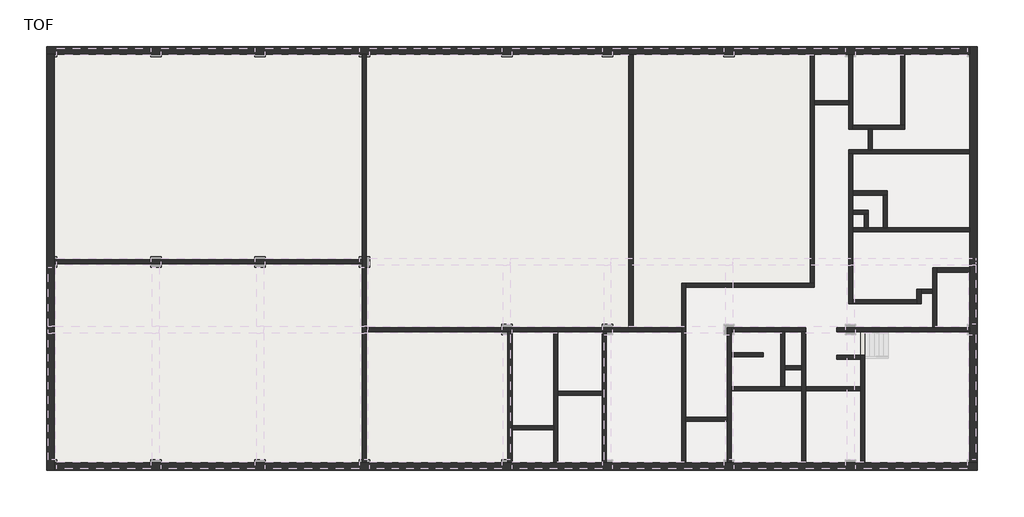
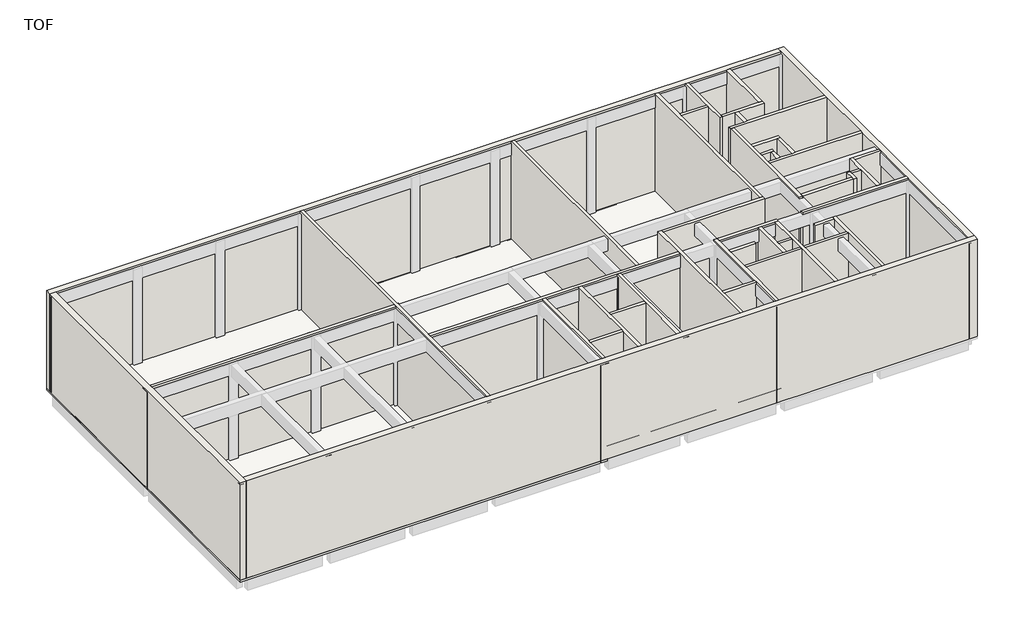
# One storey, part 1 of 3: 45 walls, 2 slabs.
"""IFC4 building model written with IfcOpenShell, lengths in millimetres."""

import ifcopenshell
import ifcopenshell.guid

model = None  # the IFC model being written
_history = None  # IfcOwnerHistory: only IFC2X3 demands one
_inside = {}  # id of a spatial element -> (the spatial element, [elements in it])
_under = {}  # id of a project, library or spatial element -> (it, [spatial elements below it])
_declared = {}  # id of a project -> (the project, [libraries it declares])
_typed = {}  # id of a type object -> (the type object, [elements of that type])
_made_of = {}  # id of a material, layer set ... -> (it, [elements and type objects made of it])


def new_model(schema):
    """Start an empty IFC model of exactly this schema.

    Asked for "IFC4X3", IfcOpenShell would pick the latest addendum, in which some entities
    have other attributes; the version numbers below select the first issue.
    IFC2X3 requires an IfcOwnerHistory on every rooted entity: one is made here for all.
    """
    global model, _history
    if schema == "IFC4X3":
        model = ifcopenshell.file(schema_version=(4, 3, 0, 0))
    else:
        model = ifcopenshell.file(schema=schema)
    _inside.clear()
    _under.clear()
    _declared.clear()
    _typed.clear()
    _made_of.clear()
    _history = None
    if model.schema == "IFC2X3":
        org = make("IfcOrganization", Name="unknown")
        user = make(
            "IfcPersonAndOrganization",
            ThePerson=make("IfcPerson", FamilyName="unknown"),
            TheOrganization=org,
        )
        app = make(
            "IfcApplication",
            ApplicationDeveloper=org,
            Version="unknown",
            ApplicationFullName="unknown",
            ApplicationIdentifier="unknown",
        )
        _history = make(
            "IfcOwnerHistory",
            OwningUser=user,
            OwningApplication=app,
            ChangeAction="ADDED",
            CreationDate=0,
        )
    return model


def make(cls, **values):
    """One entity of the class cls with the attributes given. An attribute that is None is left unset."""
    return model.create_entity(
        cls, **{name: value for name, value in values.items() if value is not None}
    )


def rooted(cls, **values):
    """An entity with a GlobalId (a new one), such as an element, a storey or a relation."""
    return make(cls, GlobalId=ifcopenshell.guid.new(), OwnerHistory=_history, **values)


def si_unit(unit_type, name, prefix=None):
    """IfcSIUnit, for example si_unit("LENGTHUNIT", "METRE", prefix="MILLI")."""
    return make("IfcSIUnit", UnitType=unit_type, Prefix=prefix, Name=name)


def assignment(units):
    """IfcUnitAssignment: the units of a project."""
    return None if units is None else make("IfcUnitAssignment", Units=units)


def point(xyz):
    """IfcCartesianPoint."""
    return None if xyz is None else make("IfcCartesianPoint", Coordinates=xyz)


def direction(xyz):
    """IfcDirection."""
    return None if xyz is None else make("IfcDirection", DirectionRatios=xyz)


def frame(location, z_axis=None, x_axis=None):
    """IfcAxis2Placement3D, a coordinate frame: its origin and axes. An axis left out is left unset."""
    return make(
        "IfcAxis2Placement3D",
        Location=point(location),
        Axis=direction(z_axis),
        RefDirection=direction(x_axis),
    )


def origin():
    """The frame at (0, 0, 0) with its axes left unset."""
    return frame((0.0, 0.0, 0.0))


def origin_with_axes():
    """The frame at (0, 0, 0) with the z axis (0, 0, 1) and the x axis (1, 0, 0) written out."""
    return frame((0.0, 0.0, 0.0), z_axis=(0.0, 0.0, 1.0), x_axis=(1.0, 0.0, 0.0))


def place(relative_to, where):
    """IfcLocalPlacement: puts the frame where relative to a parent placement (None: the world)."""
    return make(
        "IfcLocalPlacement", PlacementRelTo=relative_to, RelativePlacement=where
    )


def context(
    kind, dimensions, precision=None, world=None, true_north=None, identifier=None
):
    """IfcGeometricRepresentationContext, for example the 3D "Model" context."""
    return make(
        "IfcGeometricRepresentationContext",
        ContextIdentifier=identifier,
        ContextType=kind,
        CoordinateSpaceDimension=dimensions,
        Precision=precision,
        WorldCoordinateSystem=world,
        TrueNorth=true_north,
    )


def project(units=None, contexts=None):
    """IfcProject with its units and contexts."""
    return rooted(
        "IfcProject",
        Name="project",
        RepresentationContexts=contexts,
        UnitsInContext=assignment(units),
    )


def spatial(cls, under=None, at=None, **own):
    """A site, building, storey or space (cls), placed at a placement, below another one or the project."""
    s = rooted(cls, ObjectPlacement=at, **own)
    if under is not None:
        _under.setdefault(under.id(), (under, []))[1].append(s)
    return s


def polyline(points):
    """IfcPolyline through the points."""
    return make("IfcPolyline", Points=[point(p) for p in points])


def outline(outer, holes=None, kind="AREA"):
    """IfcArbitraryClosedProfileDef: a profile drawn as a closed curve; with holes, ...WithVoids."""
    if holes is None:
        return make("IfcArbitraryClosedProfileDef", ProfileType=kind, OuterCurve=outer)
    return make(
        "IfcArbitraryProfileDefWithVoids",
        ProfileType=kind,
        OuterCurve=outer,
        InnerCurves=holes,
    )


def extrude(swept, where, along, depth):
    """IfcExtrudedAreaSolid: the profile swept, set in the frame where, extruded along a direction by depth."""
    return make(
        "IfcExtrudedAreaSolid",
        SweptArea=swept,
        Position=where,
        ExtrudedDirection=direction(along),
        Depth=depth,
    )


def faces_of(points, faces, orient=None, outer=None):
    """IfcFace entities. A face is a list of loops; a loop is a list of indices into points, from 0.

    orient and outer hold one flag for each loop. By default every Orientation is true, the
    first loop of a face is its IfcFaceOuterBound and the others are IfcFaceBound.
    """
    made = []
    for i, loops in enumerate(faces):
        bounds = []
        for j, loop in enumerate(loops):
            is_outer = j == 0 if outer is None else outer[i][j]
            bounds.append(
                make(
                    "IfcFaceOuterBound" if is_outer else "IfcFaceBound",
                    Bound=make("IfcPolyLoop", Polygon=[points[k] for k in loop]),
                    Orientation=True if orient is None else orient[i][j],
                )
            )
        made.append(make("IfcFace", Bounds=bounds))
    return made


def faceted_brep(points, faces, orient=None, outer=None, voids=None):
    """IfcFacetedBrep: a solid bounded by flat faces; with voids (closed shells), ...WithVoids."""
    shared = [point(p) for p in points]
    hull = make("IfcClosedShell", CfsFaces=faces_of(shared, faces, orient, outer))
    if voids is None:
        return make("IfcFacetedBrep", Outer=hull)
    return make(
        "IfcFacetedBrepWithVoids",
        Outer=hull,
        Voids=[
            make(cls, CfsFaces=faces_of(shared, fs, o, b)) for cls, fs, o, b in voids
        ],
    )


def shape(context_of_items, identifier, shape_type, items):
    """IfcShapeRepresentation: the items that make up one representation, for example the "Body"."""
    return make(
        "IfcShapeRepresentation",
        ContextOfItems=context_of_items,
        RepresentationIdentifier=identifier,
        RepresentationType=shape_type,
        Items=items,
    )


def made_of(thing, what):
    """Note that an element or type object is made of a material, layer set ...; save() writes the relation."""
    if what is not None:
        _made_of.setdefault(what.id(), (what, []))[1].append(thing)
    return thing


def element(
    cls,
    number,
    at=None,
    inside=None,
    cuts=None,
    type_object=None,
    material=None,
    context=None,
    identifier="Body",
    shape_type=None,
    held_by="IfcProductDefinitionShape",
    body=None,
    shapes=None,
    **own,
):
    """One element of the class cls, such as IfcWall. Its Tag is "e" and its number.

    at: its placement. inside: the storey or other place that contains it. cuts: it is an
    opening in that element (IfcRelVoidsElement). A single representation is given by context,
    identifier, shape_type and body (its items); several are given by shapes. held_by: the class
    of the entity that holds the representations. save() writes the other relations.
    """
    e = rooted(cls, Tag="e%d" % number, ObjectPlacement=at, **own)
    if body is not None:
        shapes = [shape(context, identifier, shape_type, body)]
    if shapes is not None:
        e.Representation = make(held_by, Representations=shapes)
    if inside is not None:
        _inside.setdefault(inside.id(), (inside, []))[1].append(e)
    if cuts is not None:
        rooted(
            "IfcRelVoidsElement", RelatingBuildingElement=cuts, RelatedOpeningElement=e
        )
    if type_object is not None:
        _typed.setdefault(type_object.id(), (type_object, []))[1].append(e)
    return made_of(e, material)


def aggregate(whole, parts):
    """IfcRelAggregates: a whole, such as a stair, and the parts it consists of."""
    return rooted("IfcRelAggregates", RelatingObject=whole, RelatedObjects=parts)


def save(model, path):
    """Write the relations noted so far, then the file.

    IfcRelAggregates (storeys below a building ...), IfcRelContainedInSpatialStructure (elements
    in a storey), IfcRelDefinesByType, IfcRelAssociatesMaterial and IfcRelDeclares: one each for
    every whole, place, type object, material and project.
    """
    for whole, parts in _under.values():
        aggregate(whole, parts)
    for where, things in _inside.values():
        rooted(
            "IfcRelContainedInSpatialStructure",
            RelatedElements=things,
            RelatingStructure=where,
        )
    for kind, things in _typed.values():
        rooted("IfcRelDefinesByType", RelatedObjects=things, RelatingType=kind)
    for what, things in _made_of.values():
        rooted("IfcRelAssociatesMaterial", RelatedObjects=things, RelatingMaterial=what)
    for by, libraries in _declared.values():
        rooted("IfcRelDeclares", RelatingContext=by, RelatedDefinitions=libraries)
    model.write(path)


model = new_model("IFC4")

# Units and contexts
model_context = context("Model", 3, world=origin())
ifc_project = project(units=[si_unit("LENGTHUNIT", "METRE", prefix="MILLI")], contexts=[model_context])

# Site, building, storey
site = spatial("IfcSite", under=ifc_project)
building = spatial("IfcBuilding", under=site)
storey = spatial("IfcBuildingStorey", under=building, Name="TOF", Elevation=150.0)

# Slabs
placement = place(None, origin())
element("IfcSlab", 1, ObjectType="H_FL_AMF_RC Slab_T150", at=placement, inside=storey, context=model_context, shape_type="Brep", body=[
    faceted_brep([(-375.3, 24716.5208589, 0.0), (43724.7, 24716.5208589, 0.0), (43724.7, 10966.5208589, 0.0), (36324.7, 10966.5208589, 0.0), (36324.7, 8416.5208589, 0.0), (32224.7, 8416.5208589, 0.0), (31624.7, 8416.5208589, 0.0), (26424.7, 8416.5208589, 0.0), (25824.7, 8416.5208589, 0.0), (17924.7, 8416.5208589, 0.0), (17924.7, 12016.5208589, 0.0), (17924.7, 12316.5208589, 0.0), (17624.7, 12316.5208589, 0.0), (12224.7, 12316.5208589, 0.0), (11624.7, 12316.5208589, 0.0), (6224.7, 12316.5208589, 0.0), (5624.7, 12316.5208589, 0.0), (224.7, 12316.5208589, 0.0), (-375.3, 12316.5208589, 0.0), (-375.3, 24716.5208589, 150.0), (-375.3, 24116.5208589, 150.0), (-375.3, 12616.5208589, 150.0), (-375.3, 12316.5208589, 150.0), (224.7, 12316.5208589, 150.0), (5624.7, 12316.5208589, 150.0), (6224.7, 12316.5208589, 150.0), (11624.7, 12316.5208589, 150.0), (12224.7, 12316.5208589, 150.0), (17624.7, 12316.5208589, 150.0), (17924.7, 12316.5208589, 150.0), (17924.7, 12016.5208589, 150.0), (17924.7, 8416.5208589, 150.0), (25824.7, 8416.5208589, 150.0), (26424.7, 8416.5208589, 150.0), (31624.7, 8416.5208589, 150.0), (32224.7, 8416.5208589, 150.0), (36324.7, 8416.5208589, 150.0), (36324.7, 10966.5208589, 150.0), (43724.7, 10966.5208589, 150.0), (43724.7, 24716.5208589, 150.0), (39224.7, 24716.5208589, 150.0), (38624.7, 24716.5208589, 150.0), (32224.7, 24716.5208589, 150.0), (31624.7, 24716.5208589, 150.0), (26424.7, 24716.5208589, 150.0), (25824.7, 24716.5208589, 150.0), (18224.7, 24716.5208589, 150.0), (17624.7, 24716.5208589, 150.0), (12224.7, 24716.5208589, 150.0), (11624.7, 24716.5208589, 150.0), (6224.7, 24716.5208589, 150.0), (5624.7, 24716.5208589, 150.0), (224.7, 24716.5208589, 150.0)], [[[0, 1, 2, 3, 4, 5, 6, 7, 8, 9, 10, 11, 12, 13, 14, 15, 16, 17, 18]], [[19, 20, 21, 22, 23, 24, 25, 26, 27, 28, 29, 30, 31, 32, 33, 34, 35, 36, 37, 38, 39, 40, 41, 42, 43, 44, 45, 46, 47, 48, 49, 50, 51, 52]], [[0, 18, 22, 21, 20, 19]], [[1, 0, 19, 52, 51, 50, 49, 48, 47, 46, 45, 44, 43, 42, 41, 40, 39]], [[2, 1, 39, 38]], [[3, 2, 38, 37]], [[4, 3, 37, 36]], [[9, 8, 7, 6, 5, 4, 36, 35, 34, 33, 32, 31]], [[11, 10, 9, 31, 30, 29]], [[18, 17, 16, 15, 14, 13, 12, 11, 29, 28, 27, 26, 25, 24, 23, 22]]]),
])
element("IfcSlab", 2, ObjectType="H_FL_AMF_RC Slab_T150", at=placement, inside=storey, context=model_context, shape_type="SweptSolid", body=[
    extrude(outline(polyline([(17924.7, 12316.5208589), (17924.7, 8416.5208589), (26307.7, 8416.5208589), (26307.7, 316.5208589), (-375.3, 316.5208589), (-375.3, 12316.5208589), (17924.7, 12316.5208589)])), origin_with_axes(), (0.0, 0.0, 1.0), 150.0),
])

# Walls
element("IfcWall", 3, ObjectType="H_WA_AMW_Brick Wall_Ext (0.5B_50_1.0B / Emulsion)", at=placement, inside=storey, context=model_context, shape_type="Brep", body=[
    faceted_brep([(-375.3, 24286.5208589, 150.0), (54.7, 24286.5208589, 150.0), (17807.7, 24286.5208589, 150.0), (18041.7, 24286.5208589, 150.0), (33157.7, 24286.5208589, 150.0), (33391.7, 24286.5208589, 150.0), (43607.7, 24286.5208589, 150.0), (43841.7, 24286.5208589, 150.0), (52794.7, 24286.5208589, 150.0), (52794.7, 24286.5208589, 7650.0), (49041.7, 24286.5208589, 7650.0), (48807.7, 24286.5208589, 7650.0), (46041.7, 24286.5208589, 7650.0), (45807.7, 24286.5208589, 7650.0), (43841.7, 24286.5208589, 7650.0), (43607.7, 24286.5208589, 7650.0), (33391.7, 24286.5208589, 7650.0), (33157.7, 24286.5208589, 7650.0), (18041.7, 24286.5208589, 7650.0), (17807.7, 24286.5208589, 7650.0), (54.7, 24286.5208589, 7650.0), (-375.3, 24286.5208589, 7650.0), (-375.3, 24716.5208589, 150.0), (-375.3, 24716.5208589, 7650.0), (52794.7, 24716.5208589, 7650.0), (52794.7, 24716.5208589, 150.0)], [[[0, 1, 2, 3, 4, 5, 6, 7, 8, 9, 10, 11, 12, 13, 14, 15, 16, 17, 18, 19, 20, 21]], [[22, 23, 24, 25]], [[8, 7, 6, 5, 4, 3, 2, 1, 0, 22, 25]], [[21, 20, 19, 18, 17, 16, 15, 14, 13, 12, 11, 10, 9, 24, 23]], [[0, 21, 23, 22]], [[9, 8, 25, 24]]]),
])
element("IfcWall", 4, ObjectType="H_WA_AMW_Brick Wall_Ext (0.5B_50_1.0B / Emulsion)", at=placement, inside=storey, context=model_context, shape_type="Brep", body=[
    faceted_brep([(54.7, 316.5208589, 150.0), (54.7, 746.5208589, 150.0), (54.7, 12199.5208589, 150.0), (54.7, 12433.5208589, 150.0), (54.7, 24286.5208589, 150.0), (54.7, 24286.5208589, 7650.0), (54.7, 12433.5208589, 7650.0), (54.7, 12199.5208589, 7650.0), (54.7, 746.5208589, 7650.0), (54.7, 316.5208589, 7650.0), (-375.3, 316.5208589, 150.0), (-375.3, 316.5208589, 7650.0), (-375.3, 24286.5208589, 7650.0), (-375.3, 24286.5208589, 150.0)], [[[0, 1, 2, 3, 4, 5, 6, 7, 8, 9]], [[10, 11, 12, 13]], [[4, 3, 2, 1, 0, 10, 13]], [[9, 8, 7, 6, 5, 12, 11]], [[0, 9, 11, 10]], [[5, 4, 13, 12]]]),
])
element("IfcWall", 5, ObjectType="H_WA_AMW_Brick Wall_Ext (0.5B_50_1.0B / Emulsion)", at=placement, inside=storey, context=model_context, shape_type="Brep", body=[
    faceted_brep([(53224.7, 746.5208589, 150.0), (52794.7, 746.5208589, 150.0), (46741.7, 746.5208589, 150.0), (46507.7, 746.5208589, 150.0), (43341.7, 746.5208589, 150.0), (43107.7, 746.5208589, 150.0), (39041.7, 746.5208589, 150.0), (38807.7, 746.5208589, 150.0), (26424.7, 746.5208589, 150.0), (26190.7, 746.5208589, 150.0), (18041.7, 746.5208589, 150.0), (17807.7, 746.5208589, 150.0), (54.7, 746.5208589, 150.0), (54.7, 746.5208589, 7650.0), (17807.7, 746.5208589, 7650.0), (18041.7, 746.5208589, 7650.0), (26190.7, 746.5208589, 7650.0), (26424.7, 746.5208589, 7650.0), (28824.7, 746.5208589, 7650.0), (29058.7, 746.5208589, 7650.0), (31624.7, 746.5208589, 7650.0), (31858.7, 746.5208589, 7650.0), (36207.7, 746.5208589, 7650.0), (36441.7, 746.5208589, 7650.0), (38807.7, 746.5208589, 7650.0), (39041.7, 746.5208589, 7650.0), (43107.7, 746.5208589, 7650.0), (43341.7, 746.5208589, 7650.0), (46507.7, 746.5208589, 7650.0), (46741.7, 746.5208589, 7650.0), (52794.7, 746.5208589, 7650.0), (53224.7, 746.5208589, 7650.0), (53224.7, 316.5208589, 150.0), (53224.7, 316.5208589, 7650.0), (54.7, 316.5208589, 7650.0), (54.7, 316.5208589, 150.0)], [[[0, 1, 2, 3, 4, 5, 6, 7, 8, 9, 10, 11, 12, 13, 14, 15, 16, 17, 18, 19, 20, 21, 22, 23, 24, 25, 26, 27, 28, 29, 30, 31]], [[32, 33, 34, 35]], [[12, 11, 10, 9, 8, 7, 6, 5, 4, 3, 2, 1, 0, 32, 35]], [[31, 30, 29, 28, 27, 26, 25, 24, 23, 22, 21, 20, 19, 18, 17, 16, 15, 14, 13, 34, 33]], [[0, 31, 33, 32]], [[13, 12, 35, 34]]]),
])
element("IfcWall", 6, ObjectType="H_WA_AMW_Brick Wall_Ext (0.5B_50_1.0B / Emulsion)", at=placement, inside=storey, context=model_context, shape_type="Brep", body=[
    faceted_brep([(52794.7, 24716.5208589, 150.0), (52794.7, 24286.5208589, 150.0), (52794.7, 8533.5208589, 150.0), (52794.7, 8299.5208589, 150.0), (52794.7, 746.5208589, 150.0), (52794.7, 746.5208589, 7650.0), (52794.7, 8299.5208589, 7650.0), (52794.7, 8533.5208589, 7650.0), (52794.7, 11733.5208589, 7650.0), (52794.7, 11967.5208589, 7650.0), (52794.7, 14049.5208589, 7650.0), (52794.7, 14283.5208589, 7650.0), (52794.7, 18549.5208589, 7650.0), (52794.7, 18783.5208589, 7650.0), (52794.7, 24286.5208589, 7650.0), (52794.7, 24716.5208589, 7650.0), (53224.7, 24716.5208589, 150.0), (53224.7, 24716.5208589, 7650.0), (53224.7, 746.5208589, 7650.0), (53224.7, 746.5208589, 150.0)], [[[0, 1, 2, 3, 4, 5, 6, 7, 8, 9, 10, 11, 12, 13, 14, 15]], [[16, 17, 18, 19]], [[4, 3, 2, 1, 0, 16, 19]], [[15, 14, 13, 12, 11, 10, 9, 8, 7, 6, 5, 18, 17]], [[0, 15, 17, 16]], [[5, 4, 19, 18]]]),
])
element("IfcWall", 7, ObjectType="H_WA_AMW_Block Wall_Int_T200 (Both Plaster_Emulsion)", at=placement, inside=storey, context=model_context, shape_type="SweptSolid", body=[
    extrude(outline(polyline([(17807.7, 12199.5208589), (54.7, 12199.5208589), (54.7, 12433.5208589), (17807.7, 12433.5208589), (17807.7, 12199.5208589)])), frame((0.0, 0.0, 150.0), z_axis=(0.0, 0.0, 1.0), x_axis=(1.0, 0.0, 0.0)), (0.0, 0.0, 1.0), 7500.0),
])
element("IfcWall", 8, ObjectType="H_WA_AMW_Block Wall_Int_T200 (Both Plaster_Emulsion)", at=placement, inside=storey, context=model_context, shape_type="Brep", body=[
    faceted_brep([(17807.7, 24286.5208589, 150.0), (17807.7, 12433.5208589, 150.0), (17807.7, 12199.5208589, 150.0), (17807.7, 746.5208589, 150.0), (17807.7, 746.5208589, 7650.0), (17807.7, 12199.5208589, 7650.0), (17807.7, 12433.5208589, 7650.0), (17807.7, 24286.5208589, 7650.0), (18041.7, 24286.5208589, 150.0), (18041.7, 24286.5208589, 7650.0), (18041.7, 8533.5208589, 7650.0), (18041.7, 8299.5208589, 7650.0), (18041.7, 746.5208589, 7650.0), (18041.7, 746.5208589, 150.0), (18041.7, 8299.5208589, 150.0), (18041.7, 8533.5208589, 150.0)], [[[0, 1, 2, 3, 4, 5, 6, 7]], [[8, 9, 10, 11, 12, 13, 14, 15]], [[3, 2, 1, 0, 8, 15, 14, 13]], [[7, 6, 5, 4, 12, 11, 10, 9]], [[0, 7, 9, 8]], [[4, 3, 13, 12]]]),
])
element("IfcWall", 9, ObjectType="H_WA_AMW_Block Wall_Int_T200 (Both Plaster_Emulsion)", at=placement, inside=storey, context=model_context, shape_type="SweptSolid", body=[
    extrude(outline(polyline([(33157.7, 8533.5208589), (33157.7, 24286.5208589), (33391.7, 24286.5208589), (33391.7, 8533.5208589), (33157.7, 8533.5208589)])), frame((0.0, 0.0, 150.0), z_axis=(0.0, 0.0, 1.0), x_axis=(1.0, 0.0, 0.0)), (0.0, 0.0, 1.0), 7500.0),
])
element("IfcWall", 10, ObjectType="H_WA_AMW_Block Wall_Int_T200 (Both Plaster_Emulsion)", at=placement, inside=storey, context=model_context, shape_type="Brep", body=[
    faceted_brep([(18041.7, 8299.5208589, 150.0), (26190.7, 8299.5208589, 150.0), (26424.7, 8299.5208589, 150.0), (36207.7, 8299.5208589, 150.0), (36207.7, 8299.5208589, 7650.0), (31858.7, 8299.5208589, 7650.0), (31624.7, 8299.5208589, 7650.0), (29058.7, 8299.5208589, 7650.0), (28824.7, 8299.5208589, 7650.0), (26424.7, 8299.5208589, 7650.0), (26190.7, 8299.5208589, 7650.0), (18041.7, 8299.5208589, 7650.0), (18041.7, 8533.5208589, 150.0), (18041.7, 8533.5208589, 7650.0), (33157.7, 8533.5208589, 7650.0), (33391.7, 8533.5208589, 7650.0), (36207.7, 8533.5208589, 7650.0), (36207.7, 8533.5208589, 150.0), (33391.7, 8533.5208589, 150.0), (33157.7, 8533.5208589, 150.0)], [[[0, 1, 2, 3, 4, 5, 6, 7, 8, 9, 10, 11]], [[12, 13, 14, 15, 16, 17, 18, 19]], [[3, 2, 1, 0, 12, 19, 18, 17]], [[11, 10, 9, 8, 7, 6, 5, 4, 16, 15, 14, 13]], [[0, 11, 13, 12]], [[4, 3, 17, 16]]]),
])
element("IfcWall", 11, ObjectType="H_WA_AMW_Block Wall_Int_T200 (Both Plaster_Emulsion)", at=placement, inside=storey, context=model_context, shape_type="Brep", body=[
    faceted_brep([(36207.7, 11083.5208589, 1150.0), (36207.7, 746.5208589, 1150.0), (36207.7, 746.5208589, 7650.0), (36207.7, 8299.5208589, 7650.0), (36207.7, 8533.5208589, 7650.0), (36207.7, 11083.5208589, 7650.0), (36441.7, 11083.5208589, 1150.0), (36441.7, 11083.5208589, 7650.0), (36441.7, 10849.5208589, 7650.0), (36441.7, 3380.5208589, 7650.0), (36441.7, 3146.5208589, 7650.0), (36441.7, 746.5208589, 7650.0), (36441.7, 746.5208589, 1150.0), (36441.7, 3146.5208589, 1150.0), (36441.7, 3380.5208589, 1150.0)], [[[0, 1, 2, 3, 4, 5]], [[6, 7, 8, 9, 10, 11, 12, 13, 14]], [[1, 0, 6, 14, 13, 12]], [[5, 4, 3, 2, 11, 10, 9, 8, 7]], [[2, 1, 12, 11]], [[0, 5, 7, 6]]]),
])
element("IfcWall", 12, ObjectType="H_WA_AMW_Block Wall_Int_T200 (Both Plaster_Emulsion)", at=placement, inside=storey, context=model_context, shape_type="Brep", body=[
    faceted_brep([(36441.7, 10849.5208589, 150.0), (43841.7, 10849.5208589, 150.0), (43841.7, 10849.5208589, 7650.0), (36441.7, 10849.5208589, 7650.0), (36441.7, 11083.5208589, 150.0), (36441.7, 11083.5208589, 1150.0), (36441.7, 11083.5208589, 7650.0), (43607.7, 11083.5208589, 7650.0), (43841.7, 11083.5208589, 7650.0), (43841.7, 11083.5208589, 150.0), (43607.7, 11083.5208589, 150.0)], [[[0, 1, 2, 3]], [[4, 5, 6, 7, 8, 9, 10]], [[1, 0, 4, 10, 9]], [[3, 2, 8, 7, 6]], [[0, 3, 6, 5, 4]], [[2, 1, 9, 8]]]),
])
element("IfcWall", 13, ObjectType="H_WA_AMW_Block Wall_Int_T200 (Both Plaster_Emulsion)", at=placement, inside=storey, context=model_context, shape_type="Brep", body=[
    faceted_brep([(43841.7, 11083.5208589, 150.0), (43841.7, 24286.5208589, 150.0), (43841.7, 24286.5208589, 7650.0), (43841.7, 21586.5208589, 7650.0), (43841.7, 21352.5208589, 7650.0), (43841.7, 11083.5208589, 7650.0), (43607.7, 11083.5208589, 150.0), (43607.7, 11083.5208589, 7650.0), (43607.7, 24286.5208589, 7650.0), (43607.7, 24286.5208589, 150.0)], [[[0, 1, 2, 3, 4, 5]], [[6, 7, 8, 9]], [[1, 0, 6, 9]], [[5, 4, 3, 2, 8, 7]], [[0, 5, 7, 6]], [[2, 1, 9, 8]]]),
])
element("IfcWall", 14, ObjectType="H_WA_AMW_Block Wall_Int_T200 (Both Plaster_Emulsion)", at=placement, inside=storey, context=model_context, shape_type="SweptSolid", body=[
    extrude(outline(polyline([(45807.7, 21352.5208589), (43841.7, 21352.5208589), (43841.7, 21586.5208589), (45807.7, 21586.5208589), (45807.7, 21352.5208589)])), frame((0.0, 0.0, 1150.0), z_axis=(0.0, 0.0, 1.0), x_axis=(1.0, 0.0, 0.0)), (0.0, 0.0, 1.0), 6500.0),
])
element("IfcWall", 15, ObjectType="H_WA_AMW_Block Wall_Int_T200 (Both Plaster_Emulsion)", at=placement, inside=storey, context=model_context, shape_type="Brep", body=[
    faceted_brep([(45807.7, 24286.5208589, 1150.0), (45807.7, 21586.5208589, 1150.0), (45807.7, 21352.5208589, 1150.0), (45807.7, 19949.5208589, 1150.0), (45807.7, 19949.5208589, 7650.0), (45807.7, 21352.5208589, 7650.0), (45807.7, 21586.5208589, 7650.0), (45807.7, 24286.5208589, 7650.0), (46041.7, 24286.5208589, 1150.0), (46041.7, 24286.5208589, 7650.0), (46041.7, 20183.5208589, 7650.0), (46041.7, 19949.5208589, 7650.0), (46041.7, 19949.5208589, 1150.0), (46041.7, 20183.5208589, 1150.0)], [[[0, 1, 2, 3, 4, 5, 6, 7]], [[8, 9, 10, 11, 12, 13]], [[3, 2, 1, 0, 8, 13, 12]], [[7, 6, 5, 4, 11, 10, 9]], [[0, 7, 9, 8]], [[4, 3, 12, 11]]]),
])
element("IfcWall", 16, ObjectType="H_WA_AMW_Block Wall_Int_T200 (Both Plaster_Emulsion)", at=placement, inside=storey, context=model_context, shape_type="SweptSolid", body=[
    extrude(outline(polyline([(49743.7, 9899.5208589), (46041.7, 9899.5208589), (46041.7, 10133.5208589), (49743.7, 10133.5208589), (49743.7, 9899.5208589)])), frame((0.0, 0.0, 1150.0), z_axis=(0.0, 0.0, 1.0), x_axis=(1.0, 0.0, 0.0)), (0.0, 0.0, 1.0), 6500.0),
])
element("IfcWall", 17, ObjectType="H_WA_AMW_Block Wall_Int_T200 (Both Plaster_Emulsion)", at=placement, inside=storey, context=model_context, shape_type="Brep", body=[
    faceted_brep([(50660.7, 11967.5208589, 150.0), (50660.7, 8533.5208589, 150.0), (50660.7, 8533.5208589, 7650.0), (50660.7, 10499.5208589, 7650.0), (50660.7, 10733.5208589, 7650.0), (50660.7, 11967.5208589, 7650.0), (50894.7, 11967.5208589, 150.0), (50894.7, 11967.5208589, 1150.0), (50894.7, 11967.5208589, 7650.0), (50894.7, 11733.5208589, 7650.0), (50894.7, 8533.5208589, 7650.0), (50894.7, 8533.5208589, 150.0)], [[[0, 1, 2, 3, 4, 5]], [[6, 7, 8, 9, 10, 11]], [[1, 0, 6, 11]], [[5, 4, 3, 2, 10, 9, 8]], [[0, 5, 8, 7, 6]], [[2, 1, 11, 10]]]),
])
element("IfcWall", 18, ObjectType="H_WA_AMW_Block Wall_Int_T200 (Both Plaster_Emulsion)", at=placement, inside=storey, context=model_context, shape_type="SweptSolid", body=[
    extrude(outline(polyline([(52794.7, 11733.5208589), (50894.7, 11733.5208589), (50894.7, 11967.5208589), (52794.7, 11967.5208589), (52794.7, 11733.5208589)])), frame((0.0, 0.0, 1150.0), z_axis=(0.0, 0.0, 1.0), x_axis=(1.0, 0.0, 0.0)), (0.0, 0.0, 1.0), 6500.0),
])
element("IfcWall", 19, ObjectType="H_WA_AMW_Block Wall_Int_T200 (Both Plaster_Emulsion)", at=placement, inside=storey, context=model_context, shape_type="Brep", body=[
    faceted_brep([(49977.7, 9899.5208589, 1150.0), (49977.7, 10499.5208589, 1150.0), (49977.7, 10733.5208589, 1150.0), (49977.7, 10733.5208589, 7650.0), (49977.7, 10499.5208589, 7650.0), (49977.7, 9899.5208589, 7650.0), (49743.7, 9899.5208589, 1150.0), (49743.7, 9899.5208589, 7650.0), (49743.7, 10133.5208589, 7650.0), (49743.7, 10733.5208589, 7650.0), (49743.7, 10733.5208589, 1150.0), (49743.7, 10133.5208589, 1150.0)], [[[0, 1, 2, 3, 4, 5]], [[6, 7, 8, 9, 10, 11]], [[2, 1, 0, 6, 11, 10]], [[5, 4, 3, 9, 8, 7]], [[3, 2, 10, 9]], [[0, 5, 7, 6]]]),
])
element("IfcWall", 20, ObjectType="H_WA_AMW_Block Wall_Int_T200 (Both Plaster_Emulsion)", at=placement, inside=storey, context=model_context, shape_type="SweptSolid", body=[
    extrude(outline(polyline([(50660.7, 10499.5208589), (49977.7, 10499.5208589), (49977.7, 10733.5208589), (50660.7, 10733.5208589), (50660.7, 10499.5208589)])), frame((0.0, 0.0, 1150.0), z_axis=(0.0, 0.0, 1.0), x_axis=(1.0, 0.0, 0.0)), (0.0, 0.0, 1.0), 6500.0),
])
element("IfcWall", 21, ObjectType="H_WA_AMW_Block Wall_Int_T200 (Both Plaster_Emulsion)", at=placement, inside=storey, context=model_context, shape_type="Brep", body=[
    faceted_brep([(46507.7, 6933.5208589, 7650.0), (46507.7, 6933.5208589, 1250.0), (46507.7, 6933.5208589, 150.0), (46507.7, 6699.5208589, 150.0), (46507.7, 5130.5208589, 150.0), (46507.7, 4896.5208589, 150.0), (46507.7, 746.5208589, 150.0), (46507.7, 746.5208589, 7650.0), (46507.7, 4896.5208589, 7650.0), (46507.7, 5130.5208589, 7650.0), (46507.7, 6699.5208589, 7650.0), (46741.7, 6933.5208589, 150.0), (46741.7, 6933.5208589, 1250.0), (46741.7, 6933.5208589, 7650.0), (46741.7, 746.5208589, 7650.0), (46741.7, 746.5208589, 150.0)], [[[0, 1, 2, 3, 4, 5, 6, 7, 8, 9, 10]], [[11, 12, 13, 14, 15]], [[6, 5, 4, 3, 2, 11, 15]], [[0, 10, 9, 8, 7, 14, 13]], [[7, 6, 15, 14]], [[0, 13, 12, 11, 2, 1]]]),
])
element("IfcWall", 22, ObjectType="H_WA_AMW_Block Wall_Int_T200 (Both Plaster_Emulsion)", at=placement, inside=storey, context=model_context, shape_type="SweptSolid", body=[
    extrude(outline(polyline([(46507.7, 6699.5208589), (45124.7, 6699.5208589), (45124.7, 6933.5208589), (46507.7, 6933.5208589), (46507.7, 6699.5208589)])), frame((0.0, 0.0, 150.0), z_axis=(0.0, 0.0, 1.0), x_axis=(1.0, 0.0, 0.0)), (0.0, 0.0, 1.0), 7500.0),
])
element("IfcWall", 23, ObjectType="H_WA_AMW_Block Wall_Int_T200 (Both Plaster_Emulsion)", at=placement, inside=storey, context=model_context, shape_type="Brep", body=[
    faceted_brep([(52794.7, 8533.5208589, 150.0), (50894.7, 8533.5208589, 150.0), (50660.7, 8533.5208589, 150.0), (45124.7, 8533.5208589, 150.0), (45124.7, 8533.5208589, 7650.0), (50660.7, 8533.5208589, 7650.0), (50894.7, 8533.5208589, 7650.0), (52794.7, 8533.5208589, 7650.0), (52794.7, 8299.5208589, 150.0), (52794.7, 8299.5208589, 7650.0), (45124.7, 8299.5208589, 7650.0), (45124.7, 8299.5208589, 150.0), (46507.7, 8299.5208589, 150.0), (46741.7, 8299.5208589, 150.0)], [[[0, 1, 2, 3, 4, 5, 6, 7]], [[8, 9, 10, 11, 12, 13]], [[3, 2, 1, 0, 8, 13, 12, 11]], [[4, 3, 11, 10]], [[7, 6, 5, 4, 10, 9]], [[0, 7, 9, 8]]]),
])
element("IfcWall", 24, ObjectType="H_WA_AMW_Block Wall_Int_T200 (Both Plaster_Emulsion)", at=placement, inside=storey, context=model_context, shape_type="Brep", body=[
    faceted_brep([(38807.7, 8533.5208589, 150.0), (38807.7, 746.5208589, 150.0), (38807.7, 746.5208589, 1000.0), (38807.7, 8533.5208589, 1000.0), (38807.7, 746.5208589, 7650.0), (38807.7, 3146.5208589, 7650.0), (38807.7, 3380.5208589, 7650.0), (38807.7, 8533.5208589, 7650.0), (38807.7, 8533.5208589, 1150.0), (38807.7, 3380.5208589, 1150.0), (38807.7, 3146.5208589, 1150.0), (38807.7, 746.5208589, 1150.0), (39041.7, 746.5208589, 150.0), (39041.7, 4896.5208589, 150.0), (39041.7, 5130.5208589, 150.0), (39041.7, 6846.5208589, 150.0), (39041.7, 7080.5208589, 150.0), (39041.7, 8299.5208589, 150.0), (39041.7, 8533.5208589, 150.0), (39041.7, 8533.5208589, 1000.0), (39041.7, 8416.5208589, 1000.0), (39041.7, 8416.5208589, 1150.0), (39041.7, 8533.5208589, 1150.0), (39041.7, 8533.5208589, 7650.0), (39041.7, 8299.5208589, 7650.0), (39041.7, 7080.5208589, 7650.0), (39041.7, 6846.5208589, 7650.0), (39041.7, 5130.5208589, 7650.0), (39041.7, 4896.5208589, 7650.0), (39041.7, 746.5208589, 7650.0), (38924.7, 746.5208589, 1150.0), (38924.7, 746.5208589, 1000.0), (38924.7, 8416.5208589, 1000.0), (38924.7, 8416.5208589, 1150.0)], [[[0, 1, 2, 3]], [[4, 5, 6, 7, 8, 9, 10, 11]], [[12, 13, 14, 15, 16, 17, 18, 19, 20, 21, 22, 23, 24, 25, 26, 27, 28, 29]], [[1, 0, 18, 17, 16, 15, 14, 13, 12]], [[7, 6, 5, 4, 29, 28, 27, 26, 25, 24, 23]], [[1, 12, 29, 4, 11, 30, 31, 2]], [[7, 23, 22, 8]], [[18, 0, 3, 19]], [[31, 32, 20, 19, 3, 2]], [[21, 33, 30, 11, 10, 9, 8, 22]], [[32, 33, 21, 20]], [[33, 32, 31, 30]]]),
])
element("IfcWall", 25, ObjectType="H_WA_AMW_Block Wall_Int_T200 (Both Plaster_Emulsion)", at=placement, inside=storey, context=model_context, shape_type="Brep", body=[
    faceted_brep([(39041.7, 8299.5208589, 150.0), (41890.7, 8299.5208589, 150.0), (42124.7, 8299.5208589, 150.0), (43107.7, 8299.5208589, 150.0), (43341.7, 8299.5208589, 150.0), (43341.7, 8299.5208589, 1000.0), (43224.7, 8299.5208589, 1000.0), (43224.7, 8299.5208589, 1150.0), (43341.7, 8299.5208589, 1150.0), (43341.7, 8299.5208589, 7650.0), (43107.7, 8299.5208589, 7650.0), (42124.7, 8299.5208589, 7650.0), (41890.7, 8299.5208589, 7650.0), (39041.7, 8299.5208589, 7650.0), (43341.7, 8533.5208589, 150.0), (39041.7, 8533.5208589, 150.0), (39041.7, 8533.5208589, 1000.0), (43341.7, 8533.5208589, 1000.0), (39041.7, 8533.5208589, 7650.0), (43341.7, 8533.5208589, 7650.0), (43341.7, 8533.5208589, 1150.0), (39041.7, 8533.5208589, 1150.0), (39041.7, 8416.5208589, 1150.0), (39041.7, 8416.5208589, 1000.0), (43224.7, 8416.5208589, 1000.0), (43224.7, 8416.5208589, 1150.0)], [[[0, 1, 2, 3, 4, 5, 6, 7, 8, 9, 10, 11, 12, 13]], [[14, 15, 16, 17]], [[18, 19, 20, 21]], [[4, 3, 2, 1, 0, 15, 14]], [[13, 12, 11, 10, 9, 19, 18]], [[0, 13, 18, 21, 22, 23, 16, 15]], [[4, 14, 17, 5]], [[19, 9, 8, 20]], [[23, 24, 6, 5, 17, 16]], [[7, 25, 22, 21, 20, 8]], [[24, 25, 7, 6]], [[25, 24, 23, 22]]]),
])
element("IfcWall", 26, ObjectType="H_WA_AMW_Block Wall_Int_T200 (Both Plaster_Emulsion)", at=placement, inside=storey, context=model_context, shape_type="Brep", body=[
    faceted_brep([(43107.7, 8299.5208589, 150.0), (43107.7, 6333.5208589, 150.0), (43107.7, 6099.5208589, 150.0), (43107.7, 5130.5208589, 150.0), (43107.7, 4896.5208589, 150.0), (43107.7, 746.5208589, 150.0), (43107.7, 746.5208589, 7650.0), (43107.7, 4896.5208589, 7650.0), (43107.7, 5130.5208589, 7650.0), (43107.7, 6099.5208589, 7650.0), (43107.7, 6333.5208589, 7650.0), (43107.7, 8299.5208589, 7650.0), (43341.7, 746.5208589, 150.0), (43341.7, 4896.5208589, 150.0), (43341.7, 5130.5208589, 150.0), (43341.7, 8299.5208589, 150.0), (43341.7, 8299.5208589, 1000.0), (43341.7, 5013.5208589, 1000.0), (43341.7, 5013.5208589, 1150.0), (43341.7, 8299.5208589, 1150.0), (43341.7, 8299.5208589, 7650.0), (43341.7, 5130.5208589, 7650.0), (43341.7, 4896.5208589, 7650.0), (43341.7, 746.5208589, 7650.0), (43224.7, 8299.5208589, 1150.0), (43224.7, 8299.5208589, 1000.0), (43224.7, 5013.5208589, 1000.0), (43224.7, 5013.5208589, 1150.0)], [[[0, 1, 2, 3, 4, 5, 6, 7, 8, 9, 10, 11]], [[12, 13, 14, 15, 16, 17, 18, 19, 20, 21, 22, 23]], [[5, 4, 3, 2, 1, 0, 15, 14, 13, 12]], [[11, 10, 9, 8, 7, 6, 23, 22, 21, 20]], [[0, 11, 20, 19, 24, 25, 16, 15]], [[6, 5, 12, 23]], [[25, 26, 17, 16]], [[18, 27, 24, 19]], [[26, 27, 18, 17]], [[27, 26, 25, 24]]]),
])
element("IfcWall", 27, ObjectType="H_WA_AMW_Block Wall_Int_T200 (Both Plaster_Emulsion)", at=placement, inside=storey, context=model_context, shape_type="Brep", body=[
    faceted_brep([(39041.7, 4896.5208589, 7650.0), (39041.7, 4896.5208589, 150.0), (43107.7, 4896.5208589, 150.0), (43107.7, 4896.5208589, 7650.0), (39041.7, 5130.5208589, 150.0), (39041.7, 5130.5208589, 7650.0), (41890.7, 5130.5208589, 7650.0), (42124.7, 5130.5208589, 7650.0), (43107.7, 5130.5208589, 7650.0), (43107.7, 5130.5208589, 150.0), (42124.7, 5130.5208589, 150.0), (41890.7, 5130.5208589, 150.0)], [[[0, 1, 2, 3]], [[4, 5, 6, 7, 8, 9, 10, 11]], [[1, 4, 11, 10, 9, 2]], [[5, 0, 3, 8, 7, 6]], [[1, 0, 5, 4]], [[3, 2, 9, 8]]]),
    faceted_brep([(46507.7, 4896.5208589, 150.0), (46507.7, 4896.5208589, 7650.0), (43341.7, 4896.5208589, 7650.0), (43341.7, 4896.5208589, 150.0), (46507.7, 5130.5208589, 7650.0), (46507.7, 5130.5208589, 150.0), (43341.7, 5130.5208589, 150.0), (43341.7, 5130.5208589, 7650.0)], [[[0, 1, 2, 3]], [[4, 5, 6, 7]], [[5, 0, 3, 6]], [[1, 4, 7, 2]], [[1, 0, 5, 4]], [[3, 2, 7, 6]]]),
])
element("IfcWall", 28, ObjectType="H_WA_AMW_Block Wall_Int_T200 (Both Plaster_Emulsion)", at=placement, inside=storey, context=model_context, shape_type="SweptSolid", body=[
    extrude(outline(polyline([(40890.7, 6846.5208589), (39041.7, 6846.5208589), (39041.7, 7080.5208589), (40890.7, 7080.5208589), (40890.7, 6846.5208589)])), frame((0.0, 0.0, 150.0), z_axis=(0.0, 0.0, 1.0), x_axis=(1.0, 0.0, 0.0)), (0.0, 0.0, 1.0), 7500.0),
])
element("IfcWall", 29, ObjectType="H_WA_AMW_Block Wall_Int_T200 (Both Plaster_Emulsion)", at=placement, inside=storey, context=model_context, shape_type="Brep", body=[
    faceted_brep([(41890.7, 8299.5208589, 150.0), (41890.7, 5130.5208589, 150.0), (41890.7, 5130.5208589, 7650.0), (41890.7, 8299.5208589, 7650.0), (42124.7, 8299.5208589, 150.0), (42124.7, 8299.5208589, 7650.0), (42124.7, 6333.5208589, 7650.0), (42124.7, 6099.5208589, 7650.0), (42124.7, 5130.5208589, 7650.0), (42124.7, 5130.5208589, 150.0), (42124.7, 6099.5208589, 150.0), (42124.7, 6333.5208589, 150.0)], [[[0, 1, 2, 3]], [[4, 5, 6, 7, 8, 9, 10, 11]], [[1, 0, 4, 11, 10, 9]], [[3, 2, 8, 7, 6, 5]], [[0, 3, 5, 4]], [[2, 1, 9, 8]]]),
])
element("IfcWall", 30, ObjectType="H_WA_AMW_Block Wall_Int_T200 (Both Plaster_Emulsion)", at=placement, inside=storey, context=model_context, shape_type="SweptSolid", body=[
    extrude(outline(polyline([(43107.7, 6099.5208589), (42124.7, 6099.5208589), (42124.7, 6333.5208589), (43107.7, 6333.5208589), (43107.7, 6099.5208589)])), frame((0.0, 0.0, 150.0), z_axis=(0.0, 0.0, 1.0), x_axis=(1.0, 0.0, 0.0)), (0.0, 0.0, 1.0), 7500.0),
])
element("IfcWall", 31, ObjectType="H_WA_AMW_Block Wall_Int_T200 (Both Plaster_Emulsion)", at=placement, inside=storey, context=model_context, shape_type="Brep", body=[
    faceted_brep([(31624.7, 8299.5208589, 1150.0), (31624.7, 4880.5208589, 1150.0), (31624.7, 4646.5208589, 1150.0), (31624.7, 746.5208589, 1150.0), (31624.7, 746.5208589, 7650.0), (31624.7, 4646.5208589, 7650.0), (31624.7, 4880.5208589, 7650.0), (31624.7, 8299.5208589, 7650.0), (31858.7, 8299.5208589, 1150.0), (31858.7, 8299.5208589, 7650.0), (31858.7, 746.5208589, 7650.0), (31858.7, 746.5208589, 1150.0)], [[[0, 1, 2, 3, 4, 5, 6, 7]], [[8, 9, 10, 11]], [[3, 2, 1, 0, 8, 11]], [[7, 6, 5, 4, 10, 9]], [[0, 7, 9, 8]], [[4, 3, 11, 10]]]),
])
element("IfcWall", 32, ObjectType="H_WA_AMW_Block Wall_Int_T200 (Both Plaster_Emulsion)", at=placement, inside=storey, context=model_context, shape_type="Brep", body=[
    faceted_brep([(28824.7, 8299.5208589, 1150.0), (28824.7, 2880.5208589, 1150.0), (28824.7, 2646.5208589, 1150.0), (28824.7, 746.5208589, 1150.0), (28824.7, 746.5208589, 7650.0), (28824.7, 2646.5208589, 7650.0), (28824.7, 2880.5208589, 7650.0), (28824.7, 8299.5208589, 7650.0), (29058.7, 8299.5208589, 1150.0), (29058.7, 8299.5208589, 7650.0), (29058.7, 4880.5208589, 7650.0), (29058.7, 4646.5208589, 7650.0), (29058.7, 746.5208589, 7650.0), (29058.7, 746.5208589, 1150.0), (29058.7, 4646.5208589, 1150.0), (29058.7, 4880.5208589, 1150.0)], [[[0, 1, 2, 3, 4, 5, 6, 7]], [[8, 9, 10, 11, 12, 13, 14, 15]], [[3, 2, 1, 0, 8, 15, 14, 13]], [[7, 6, 5, 4, 12, 11, 10, 9]], [[4, 3, 13, 12]], [[0, 7, 9, 8]]]),
])
element("IfcWall", 33, ObjectType="H_WA_AMW_Block Wall_Int_T200 (Both Plaster_Emulsion)", at=placement, inside=storey, context=model_context, shape_type="Brep", body=[
    faceted_brep([(26190.7, 8299.5208589, 150.0), (26190.7, 746.5208589, 150.0), (26190.7, 746.5208589, 7650.0), (26190.7, 8299.5208589, 7650.0), (26424.7, 8299.5208589, 150.0), (26424.7, 8299.5208589, 7650.0), (26424.7, 2880.5208589, 7650.0), (26424.7, 2646.5208589, 7650.0), (26424.7, 746.5208589, 7650.0), (26424.7, 746.5208589, 150.0)], [[[0, 1, 2, 3]], [[4, 5, 6, 7, 8, 9]], [[1, 0, 4, 9]], [[3, 2, 8, 7, 6, 5]], [[2, 1, 9, 8]], [[0, 3, 5, 4]]]),
])
element("IfcWall", 34, ObjectType="H_WA_AMW_Block Wall_Int_T200 (Both Plaster_Emulsion)", at=placement, inside=storey, context=model_context, shape_type="SweptSolid", body=[
    extrude(outline(polyline([(31624.7, 4646.5208589), (29058.7, 4646.5208589), (29058.7, 4880.5208589), (31624.7, 4880.5208589), (31624.7, 4646.5208589)])), frame((0.0, 0.0, 1150.0), z_axis=(0.0, 0.0, 1.0), x_axis=(1.0, 0.0, 0.0)), (0.0, 0.0, 1.0), 6500.0),
])
element("IfcWall", 35, ObjectType="H_WA_AMW_Block Wall_Int_T200 (Both Plaster_Emulsion)", at=placement, inside=storey, context=model_context, shape_type="SweptSolid", body=[
    extrude(outline(polyline([(28824.7, 2646.5208589), (26424.7, 2646.5208589), (26424.7, 2880.5208589), (28824.7, 2880.5208589), (28824.7, 2646.5208589)])), frame((0.0, 0.0, 1150.0), z_axis=(0.0, 0.0, 1.0), x_axis=(1.0, 0.0, 0.0)), (0.0, 0.0, 1.0), 6500.0),
])
element("IfcWall", 36, ObjectType="H_WA_AMW_Block Wall_Int_T200 (Both Plaster_Emulsion)", at=placement, inside=storey, context=model_context, shape_type="Brep", body=[
    faceted_brep([(45807.7, 18549.5208589, 1150.0), (46041.7, 18549.5208589, 1150.0), (52794.7, 18549.5208589, 1150.0), (52794.7, 18549.5208589, 7650.0), (46041.7, 18549.5208589, 7650.0), (45807.7, 18549.5208589, 7650.0), (45807.7, 18783.5208589, 1150.0), (45807.7, 18783.5208589, 7650.0), (46924.7, 18783.5208589, 7650.0), (47158.7, 18783.5208589, 7650.0), (52794.7, 18783.5208589, 7650.0), (52794.7, 18783.5208589, 1150.0), (47158.7, 18783.5208589, 1150.0), (46924.7, 18783.5208589, 1150.0)], [[[0, 1, 2, 3, 4, 5]], [[6, 7, 8, 9, 10, 11, 12, 13]], [[2, 1, 0, 6, 13, 12, 11]], [[5, 4, 3, 10, 9, 8, 7]], [[3, 2, 11, 10]], [[0, 5, 7, 6]]]),
])
element("IfcWall", 37, ObjectType="H_WA_AMW_Block Wall_Int_T200 (Both Plaster_Emulsion)", at=placement, inside=storey, context=model_context, shape_type="SweptSolid", body=[
    extrude(outline(polyline([(38807.7, 3146.5208589), (36441.7, 3146.5208589), (36441.7, 3380.5208589), (38807.7, 3380.5208589), (38807.7, 3146.5208589)])), frame((0.0, 0.0, 1150.0), z_axis=(0.0, 0.0, 1.0), x_axis=(1.0, 0.0, 0.0)), (0.0, 0.0, 1.0), 6500.0),
])
element("IfcWall", 38, ObjectType="H_WA_AMW_Block Wall_Int_T200 (Both Plaster_Emulsion)", at=placement, inside=storey, context=model_context, shape_type="Brep", body=[
    faceted_brep([(46041.7, 19949.5208589, 1150.0), (46924.7, 19949.5208589, 1150.0), (47158.7, 19949.5208589, 1150.0), (49041.7, 19949.5208589, 1150.0), (49041.7, 19949.5208589, 7650.0), (47158.7, 19949.5208589, 7650.0), (46924.7, 19949.5208589, 7650.0), (46041.7, 19949.5208589, 7650.0), (46041.7, 20183.5208589, 1150.0), (46041.7, 20183.5208589, 7650.0), (48807.7, 20183.5208589, 7650.0), (49041.7, 20183.5208589, 7650.0), (49041.7, 20183.5208589, 1150.0), (48807.7, 20183.5208589, 1150.0)], [[[0, 1, 2, 3, 4, 5, 6, 7]], [[8, 9, 10, 11, 12, 13]], [[3, 2, 1, 0, 8, 13, 12]], [[7, 6, 5, 4, 11, 10, 9]], [[4, 3, 12, 11]], [[0, 7, 9, 8]]]),
])
element("IfcWall", 39, ObjectType="H_WA_AMW_Block Wall_Int_T200 (Both Plaster_Emulsion)", at=placement, inside=storey, context=model_context, shape_type="SweptSolid", body=[
    extrude(outline(polyline([(48807.7, 20183.5208589), (48807.7, 24286.5208589), (49041.7, 24286.5208589), (49041.7, 20183.5208589), (48807.7, 20183.5208589)])), frame((0.0, 0.0, 1150.0), z_axis=(0.0, 0.0, 1.0), x_axis=(1.0, 0.0, 0.0)), (0.0, 0.0, 1.0), 6500.0),
])
element("IfcWall", 40, ObjectType="H_WA_AMW_Block Wall_Int_T200 (Both Plaster_Emulsion)", at=placement, inside=storey, context=model_context, shape_type="Brep", body=[
    faceted_brep([(45807.7, 18549.5208589, 1150.0), (45807.7, 9899.5208589, 1150.0), (45807.7, 9899.5208589, 7650.0), (45807.7, 18549.5208589, 7650.0), (46041.7, 18549.5208589, 1150.0), (46041.7, 18549.5208589, 7650.0), (46041.7, 16400.5208589, 7650.0), (46041.7, 16166.5208589, 7650.0), (46041.7, 15300.5208589, 7650.0), (46041.7, 15066.5208589, 7650.0), (46041.7, 14283.5208589, 7650.0), (46041.7, 14049.5208589, 7650.0), (46041.7, 10133.5208589, 7650.0), (46041.7, 9899.5208589, 7650.0), (46041.7, 9899.5208589, 1150.0), (46041.7, 10133.5208589, 1150.0), (46041.7, 14049.5208589, 1150.0), (46041.7, 14283.5208589, 1150.0), (46041.7, 15066.5208589, 1150.0), (46041.7, 15300.5208589, 1150.0), (46041.7, 16166.5208589, 1150.0), (46041.7, 16400.5208589, 1150.0)], [[[0, 1, 2, 3]], [[4, 5, 6, 7, 8, 9, 10, 11, 12, 13, 14, 15, 16, 17, 18, 19, 20, 21]], [[1, 0, 4, 21, 20, 19, 18, 17, 16, 15, 14]], [[3, 2, 13, 12, 11, 10, 9, 8, 7, 6, 5]], [[2, 1, 14, 13]], [[0, 3, 5, 4]]]),
])
element("IfcWall", 41, ObjectType="H_WA_AMW_Block Wall_Int_T200 (Both Plaster_Emulsion)", at=placement, inside=storey, context=model_context, shape_type="SweptSolid", body=[
    extrude(outline(polyline([(46924.7, 18783.5208589), (46924.7, 19949.5208589), (47158.7, 19949.5208589), (47158.7, 18783.5208589), (46924.7, 18783.5208589)])), frame((0.0, 0.0, 1150.0), z_axis=(0.0, 0.0, 1.0), x_axis=(1.0, 0.0, 0.0)), (0.0, 0.0, 1.0), 6500.0),
])
element("IfcWall", 42, ObjectType="H_WA_AMW_Block Wall_Int_T200 (Both Plaster_Emulsion)", at=placement, inside=storey, context=model_context, shape_type="Brep", body=[
    faceted_brep([(46041.7, 14049.5208589, 1150.0), (52794.7, 14049.5208589, 1150.0), (52794.7, 14049.5208589, 7650.0), (46041.7, 14049.5208589, 7650.0), (46041.7, 14283.5208589, 1150.0), (46041.7, 14283.5208589, 7650.0), (46707.7, 14283.5208589, 7650.0), (46941.7, 14283.5208589, 7650.0), (47807.7, 14283.5208589, 7650.0), (48041.7, 14283.5208589, 7650.0), (52794.7, 14283.5208589, 7650.0), (52794.7, 14283.5208589, 1150.0), (48041.7, 14283.5208589, 1150.0), (47807.7, 14283.5208589, 1150.0), (46941.7, 14283.5208589, 1150.0), (46707.7, 14283.5208589, 1150.0)], [[[0, 1, 2, 3]], [[4, 5, 6, 7, 8, 9, 10, 11, 12, 13, 14, 15]], [[1, 0, 4, 15, 14, 13, 12, 11]], [[3, 2, 10, 9, 8, 7, 6, 5]], [[2, 1, 11, 10]], [[0, 3, 5, 4]]]),
])
element("IfcWall", 43, ObjectType="H_WA_AMW_Block Wall_Int_T200 (Both Plaster_Emulsion)", at=placement, inside=storey, context=model_context, shape_type="Brep", body=[
    faceted_brep([(46041.7, 16166.5208589, 1150.0), (47807.7, 16166.5208589, 1150.0), (48041.7, 16166.5208589, 1150.0), (48041.7, 16166.5208589, 7650.0), (47807.7, 16166.5208589, 7650.0), (46041.7, 16166.5208589, 7650.0), (46041.7, 16400.5208589, 1150.0), (46041.7, 16400.5208589, 7650.0), (48041.7, 16400.5208589, 7650.0), (48041.7, 16400.5208589, 1150.0)], [[[0, 1, 2, 3, 4, 5]], [[6, 7, 8, 9]], [[2, 1, 0, 6, 9]], [[5, 4, 3, 8, 7]], [[0, 5, 7, 6]], [[3, 2, 9, 8]]]),
])
element("IfcWall", 44, ObjectType="H_WA_AMW_Block Wall_Int_T200 (Both Plaster_Emulsion)", at=placement, inside=storey, context=model_context, shape_type="SweptSolid", body=[
    extrude(outline(polyline([(47807.7, 14283.5208589), (47807.7, 16166.5208589), (48041.7, 16166.5208589), (48041.7, 14283.5208589), (47807.7, 14283.5208589)])), frame((0.0, 0.0, 1150.0), z_axis=(0.0, 0.0, 1.0), x_axis=(1.0, 0.0, 0.0)), (0.0, 0.0, 1.0), 6500.0),
])
element("IfcWall", 45, ObjectType="H_WA_AMW_Block Wall_Int_T200 (Both Plaster_Emulsion)", at=placement, inside=storey, context=model_context, shape_type="Brep", body=[
    faceted_brep([(46041.7, 15066.5208589, 1150.0), (46707.7, 15066.5208589, 1150.0), (46941.7, 15066.5208589, 1150.0), (46941.7, 15066.5208589, 7650.0), (46707.7, 15066.5208589, 7650.0), (46041.7, 15066.5208589, 7650.0), (46041.7, 15300.5208589, 1150.0), (46041.7, 15300.5208589, 7650.0), (46941.7, 15300.5208589, 7650.0), (46941.7, 15300.5208589, 1150.0)], [[[0, 1, 2, 3, 4, 5]], [[6, 7, 8, 9]], [[2, 1, 0, 6, 9]], [[5, 4, 3, 8, 7]], [[0, 5, 7, 6]], [[3, 2, 9, 8]]]),
])
element("IfcWall", 46, ObjectType="H_WA_AMW_Block Wall_Int_T200 (Both Plaster_Emulsion)", at=placement, inside=storey, context=model_context, shape_type="SweptSolid", body=[
    extrude(outline(polyline([(46707.7, 14283.5208589), (46707.7, 15066.5208589), (46941.7, 15066.5208589), (46941.7, 14283.5208589), (46707.7, 14283.5208589)])), frame((0.0, 0.0, 1150.0), z_axis=(0.0, 0.0, 1.0), x_axis=(1.0, 0.0, 0.0)), (0.0, 0.0, 1.0), 6500.0),
])
element("IfcWall", 47, ObjectType="H_WA_AMW_Block Wall_Int_T200 (Both Plaster_Emulsion)", at=placement, inside=storey, context=model_context, shape_type="SweptSolid", body=[
    extrude(outline(polyline([(46507.7, 6933.5208589), (46507.7, 8299.5208589), (46741.7, 8299.5208589), (46741.7, 6933.5208589), (46507.7, 6933.5208589)])), frame((0.0, 0.0, 150.0), z_axis=(0.0, 0.0, 1.0), x_axis=(1.0, 0.0, 0.0)), (0.0, 0.0, 1.0), 1100.0),
])

save(model, "model.ifc")

# Revit data of these elements
# Project information
#   Project Status = "Project Status"
#   Client Name = "현대엔지니어링"
#   Project Address = "서울시 종로구 율곡로 75(계동)"
#   Project Number = "-"
# Grids (mm)
#   "Y1": line (-3935.398, 24416.521) -> (58968.688, 24416.521)
#   "X1": line (-75.3, 29394.337) -> (-75.3, -4379.638)
#   "X2": line (5924.7, 29394.337) -> (5924.7, -4379.638)
#   "Y3": line (-3935.398, 8416.521) -> (58968.688, 8416.521)
#   "Y4": line (-3935.398, 616.521) -> (58968.688, 616.521)
#   "X3": line (11924.7, 29394.337) -> (11924.7, -4379.638)
#   "X4": line (17924.7, 29394.337) -> (17924.7, -4379.638)
#   "X5": line (26124.7, 29394.337) -> (26124.7, -4379.638)
#   "X6": line (31924.7, 29394.337) -> (31924.7, -4379.638)
#   "X7": line (38924.7, 29394.337) -> (38924.7, -4379.638)
#   "X8": line (45924.7, 29394.337) -> (45924.7, -4379.638)
#   "X9": line (52924.7, 29394.337) -> (52924.7, -4379.638)
#   "X15": line (43724.7, 27041.858) -> (43724.7, 9156.488)
#   "X16": line (36324.7, 27041.858) -> (36324.7, 9156.488)
#   "X17": line (34685.051, 10966.521) -> (55094.626, 10966.521)
#   "X18": line (34685.051, 18666.521) -> (55094.626, 18666.521)
#   "Y2": line (-3935.398, 12316.521) -> (58968.688, 12316.521)
# Type "H_FL_AMF_RC Slab_T150"
#   Keynote = ""
#   Type Comments = ""
#   Description = ""
#   Function = 1
#   Layers, outside or top first: 150.000 mm no material (function 1)
# Type "H_WA_AMW_Brick Wall_Ext (0.5B_50_1.0B / Emulsion)"
#   Type Comments = ""
#   Layers, outside or top first: 0.000 mm no material (function 100); 20.000 mm no material (function 2); 115.000 mm no material (function 1); 50.000 mm no material (function 3); 0.000 mm no material (function 100); 230.000 mm no material (function 1); 15.000 mm no material (function 2); 0.000 mm no material (function 100); 0.000 mm no material (function 100)
# Type "H_WA_AMW_Block Wall_Int_T200 (Both Plaster_Emulsion)"
#   Type Comments = ""
#   Layers, outside or top first: 0.000 mm no material (function 100); 12.000 mm no material (function 2); 200.000 mm no material (function 1); 12.000 mm no material (function 2); 10.000 mm no material (function 5)
# Element 1 (IfcSlab, "H_FL_AMF_RC Slab_T150")
#   Height Offset From Level = 0.000 mm
#   Phase Created = New Construction
#   Materials on its faces: "Default Floor"
# Element 2 (IfcSlab, "H_FL_AMF_RC Slab_T150")
#   built-in parameter 1001955 = 1.5708 (stored number, unit not read)
#   Height Offset From Level = 0.000 mm
#   Phase Created = New Construction
#   Materials on its faces: "Default Floor"
# Elements 3, 4, 5, 6 (IfcWall, "H_WA_AMW_Brick Wall_Ext (0.5B_50_1.0B / Emulsion)")
#   Top Offset = 0.000 mm
#   Base Offset = 0.000 mm
#   wall height = 7500.000 mm
#   Phase Created = New Construction
#   Base Constraint = TOF
#   Top Constraint = TOC
#   Materials on its faces: "Default Wall"
# Elements 7, 8, 9, 10, 12, 13, 17, 21, 22, 23, 24, 25, 26, 27, 28, 29, 30, 33 (IfcWall, "H_WA_AMW_Block Wall_Int_T200 (Both Plaster_Emulsion)")
#   Top Offset = 0.000 mm
#   Base Offset = 0.000 mm
#   wall height = 7500.000 mm
#   Phase Created = New Construction
#   Base Constraint = TOF
#   Top Constraint = TOC
#   Materials on its faces: "Default Wall"
# Elements 11, 14, 15, 16, 18, 19, 20, 31, 32, 34, 35, 36, 37, 38, 39, 40, 41, 42, 43, 44, 45, 46 (IfcWall, "H_WA_AMW_Block Wall_Int_T200 (Both Plaster_Emulsion)")
#   built-in parameter 1001111 = 1000.000 mm
#   Top Offset = 0.000 mm
#   Base Offset = 1000.000 mm
#   wall height = 6500.000 mm
#   Phase Created = New Construction
#   Base Constraint = TOF
#   Top Constraint = TOC
#   Materials on its faces: "Default Wall"
# Element 47 (IfcWall, "H_WA_AMW_Block Wall_Int_T200 (Both Plaster_Emulsion)")
#   Top Offset = 0.000 mm
#   Base Offset = 0.000 mm
#   Unconnected Height = 1100.000 mm
#   wall height = 1100.000 mm
#   Phase Created = New Construction
#   Base Constraint = TOF
#   Materials on its faces: "Default Wall"
# Materials
#   "Default Floor": class "Miscellaneous", colour RGB 80 80 80, transparency 0
#   "Default Wall": class "Miscellaneous", colour RGB 80 80 80, transparency 0
